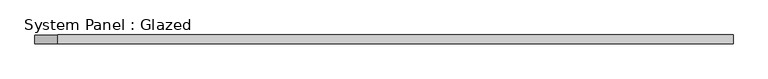
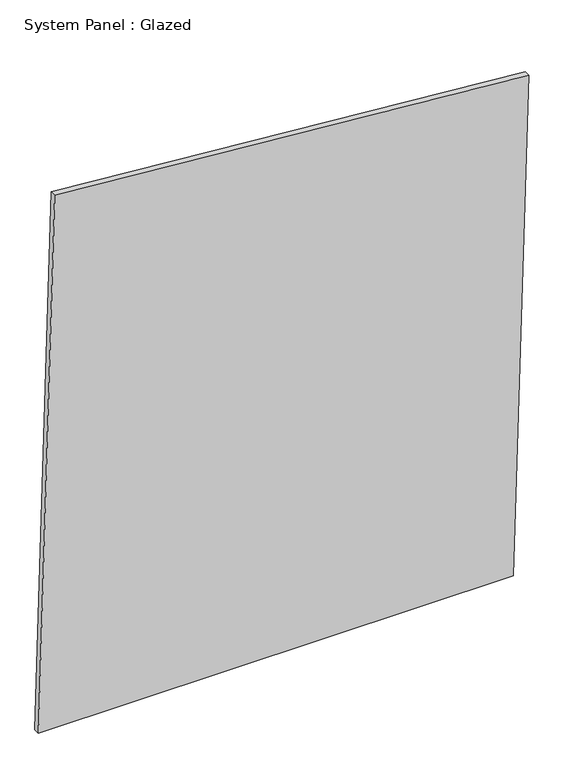
"""IFC4 building model written with IfcOpenShell, lengths in millimetres: plate geometry, System Panel : Glazed."""

import ifcopenshell
import ifcopenshell.guid

model = None  # the IFC model being written
_history = None  # IfcOwnerHistory: only IFC2X3 demands one
_inside = {}  # id of a spatial element -> (the spatial element, [elements in it])
_under = {}  # id of a project, library or spatial element -> (it, [spatial elements below it])
_declared = {}  # id of a project -> (the project, [libraries it declares])
_typed = {}  # id of a type object -> (the type object, [elements of that type])
_made_of = {}  # id of a material, layer set ... -> (it, [elements and type objects made of it])


def new_model(schema):
    """Start an empty IFC model of exactly this schema.

    Asked for "IFC4X3", IfcOpenShell would pick the latest addendum, in which some entities
    have other attributes; the version numbers below select the first issue.
    IFC2X3 requires an IfcOwnerHistory on every rooted entity: one is made here for all.
    """
    global model, _history
    if schema == "IFC4X3":
        model = ifcopenshell.file(schema_version=(4, 3, 0, 0))
    else:
        model = ifcopenshell.file(schema=schema)
    _inside.clear()
    _under.clear()
    _declared.clear()
    _typed.clear()
    _made_of.clear()
    _history = None
    if model.schema == "IFC2X3":
        org = make("IfcOrganization", Name="unknown")
        user = make(
            "IfcPersonAndOrganization",
            ThePerson=make("IfcPerson", FamilyName="unknown"),
            TheOrganization=org,
        )
        app = make(
            "IfcApplication",
            ApplicationDeveloper=org,
            Version="unknown",
            ApplicationFullName="unknown",
            ApplicationIdentifier="unknown",
        )
        _history = make(
            "IfcOwnerHistory",
            OwningUser=user,
            OwningApplication=app,
            ChangeAction="ADDED",
            CreationDate=0,
        )
    return model


def make(cls, **values):
    """One entity of the class cls with the attributes given. An attribute that is None is left unset."""
    return model.create_entity(
        cls, **{name: value for name, value in values.items() if value is not None}
    )


def rooted(cls, **values):
    """An entity with a GlobalId (a new one), such as an element, a storey or a relation."""
    return make(cls, GlobalId=ifcopenshell.guid.new(), OwnerHistory=_history, **values)


def si_unit(unit_type, name, prefix=None):
    """IfcSIUnit, for example si_unit("LENGTHUNIT", "METRE", prefix="MILLI")."""
    return make("IfcSIUnit", UnitType=unit_type, Prefix=prefix, Name=name)


def assignment(units):
    """IfcUnitAssignment: the units of a project."""
    return None if units is None else make("IfcUnitAssignment", Units=units)


def point(xyz):
    """IfcCartesianPoint."""
    return None if xyz is None else make("IfcCartesianPoint", Coordinates=xyz)


def direction(xyz):
    """IfcDirection."""
    return None if xyz is None else make("IfcDirection", DirectionRatios=xyz)


def frame(location, z_axis=None, x_axis=None):
    """IfcAxis2Placement3D, a coordinate frame: its origin and axes. An axis left out is left unset."""
    return make(
        "IfcAxis2Placement3D",
        Location=point(location),
        Axis=direction(z_axis),
        RefDirection=direction(x_axis),
    )


def origin():
    """The frame at (0, 0, 0) with its axes left unset."""
    return frame((0.0, 0.0, 0.0))


def place(relative_to, where):
    """IfcLocalPlacement: puts the frame where relative to a parent placement (None: the world)."""
    return make(
        "IfcLocalPlacement", PlacementRelTo=relative_to, RelativePlacement=where
    )


def context(
    kind, dimensions, precision=None, world=None, true_north=None, identifier=None
):
    """IfcGeometricRepresentationContext, for example the 3D "Model" context."""
    return make(
        "IfcGeometricRepresentationContext",
        ContextIdentifier=identifier,
        ContextType=kind,
        CoordinateSpaceDimension=dimensions,
        Precision=precision,
        WorldCoordinateSystem=world,
        TrueNorth=true_north,
    )


def project(units=None, contexts=None):
    """IfcProject with its units and contexts."""
    return rooted(
        "IfcProject",
        Name="project",
        RepresentationContexts=contexts,
        UnitsInContext=assignment(units),
    )


def spatial(cls, under=None, at=None, **own):
    """A site, building, storey or space (cls), placed at a placement, below another one or the project."""
    s = rooted(cls, ObjectPlacement=at, **own)
    if under is not None:
        _under.setdefault(under.id(), (under, []))[1].append(s)
    return s


def polyline(points):
    """IfcPolyline through the points."""
    return make("IfcPolyline", Points=[point(p) for p in points])


def outline(outer, holes=None, kind="AREA"):
    """IfcArbitraryClosedProfileDef: a profile drawn as a closed curve; with holes, ...WithVoids."""
    if holes is None:
        return make("IfcArbitraryClosedProfileDef", ProfileType=kind, OuterCurve=outer)
    return make(
        "IfcArbitraryProfileDefWithVoids",
        ProfileType=kind,
        OuterCurve=outer,
        InnerCurves=holes,
    )


def extrude(swept, where, along, depth):
    """IfcExtrudedAreaSolid: the profile swept, set in the frame where, extruded along a direction by depth."""
    return make(
        "IfcExtrudedAreaSolid",
        SweptArea=swept,
        Position=where,
        ExtrudedDirection=direction(along),
        Depth=depth,
    )


def shape(context_of_items, identifier, shape_type, items):
    """IfcShapeRepresentation: the items that make up one representation, for example the "Body"."""
    return make(
        "IfcShapeRepresentation",
        ContextOfItems=context_of_items,
        RepresentationIdentifier=identifier,
        RepresentationType=shape_type,
        Items=items,
    )


def source(mapping_origin, context_of_items, identifier, shape_type, items):
    """IfcRepresentationMap: a shape defined once, which mapped items show again and again."""
    return make(
        "IfcRepresentationMap",
        MappingOrigin=mapping_origin,
        MappedRepresentation=shape(context_of_items, identifier, shape_type, items),
    )


def transform(
    local_origin,
    x_axis=None,
    y_axis=None,
    z_axis=None,
    scale=None,
    scale2=None,
    scale3=None,
    uniform=True,
):
    """IfcCartesianTransformationOperator3D, or its non-uniform kind. x_axis, y_axis, z_axis: its Axis1, 2, 3."""
    if uniform:
        return make(
            "IfcCartesianTransformationOperator3D",
            Axis1=direction(x_axis),
            Axis2=direction(y_axis),
            LocalOrigin=point(local_origin),
            Scale=scale,
            Axis3=direction(z_axis),
        )
    return make(
        "IfcCartesianTransformationOperator3DnonUniform",
        Axis1=direction(x_axis),
        Axis2=direction(y_axis),
        LocalOrigin=point(local_origin),
        Scale=scale,
        Axis3=direction(z_axis),
        Scale2=scale2,
        Scale3=scale3,
    )


def mapped(mapping_source, mapping_target):
    """IfcMappedItem: shows the shape of a source again, moved by a transform."""
    return make(
        "IfcMappedItem", MappingSource=mapping_source, MappingTarget=mapping_target
    )


def made_of(thing, what):
    """Note that an element or type object is made of a material, layer set ...; save() writes the relation."""
    if what is not None:
        _made_of.setdefault(what.id(), (what, []))[1].append(thing)
    return thing


def element(
    cls,
    number,
    at=None,
    inside=None,
    cuts=None,
    type_object=None,
    material=None,
    context=None,
    identifier="Body",
    shape_type=None,
    held_by="IfcProductDefinitionShape",
    body=None,
    shapes=None,
    **own,
):
    """One element of the class cls, such as IfcWall. Its Tag is "e" and its number.

    at: its placement. inside: the storey or other place that contains it. cuts: it is an
    opening in that element (IfcRelVoidsElement). A single representation is given by context,
    identifier, shape_type and body (its items); several are given by shapes. held_by: the class
    of the entity that holds the representations. save() writes the other relations.
    """
    e = rooted(cls, Tag="e%d" % number, ObjectPlacement=at, **own)
    if body is not None:
        shapes = [shape(context, identifier, shape_type, body)]
    if shapes is not None:
        e.Representation = make(held_by, Representations=shapes)
    if inside is not None:
        _inside.setdefault(inside.id(), (inside, []))[1].append(e)
    if cuts is not None:
        rooted(
            "IfcRelVoidsElement", RelatingBuildingElement=cuts, RelatedOpeningElement=e
        )
    if type_object is not None:
        _typed.setdefault(type_object.id(), (type_object, []))[1].append(e)
    return made_of(e, material)


def aggregate(whole, parts):
    """IfcRelAggregates: a whole, such as a stair, and the parts it consists of."""
    return rooted("IfcRelAggregates", RelatingObject=whole, RelatedObjects=parts)


def save(model, path):
    """Write the relations noted so far, then the file.

    IfcRelAggregates (storeys below a building ...), IfcRelContainedInSpatialStructure (elements
    in a storey), IfcRelDefinesByType, IfcRelAssociatesMaterial and IfcRelDeclares: one each for
    every whole, place, type object, material and project.
    """
    for whole, parts in _under.values():
        aggregate(whole, parts)
    for where, things in _inside.values():
        rooted(
            "IfcRelContainedInSpatialStructure",
            RelatedElements=things,
            RelatingStructure=where,
        )
    for kind, things in _typed.values():
        rooted("IfcRelDefinesByType", RelatedObjects=things, RelatingType=kind)
    for what, things in _made_of.values():
        rooted("IfcRelAssociatesMaterial", RelatedObjects=things, RelatingMaterial=what)
    for by, libraries in _declared.values():
        rooted("IfcRelDeclares", RelatingContext=by, RelatedDefinitions=libraries)
    model.write(path)


def system_panel_glazed_15b89219(model_context):
    return source(origin(), model_context, "Body", "SweptSolid", [
        extrude(outline(polyline([(0.0, -1007.0351176), (0.0, 942.9445704), (2151.1749822, 1007.0351176), (2310.4173325, -940.4629834), (0.0, -1007.0351176)])), frame((0.0, -49.5, 0.0), z_axis=(0.0, 1.0, 0.0), x_axis=(0.0, 0.0, 1.0)), (0.0, 0.0, 1.0), 25.0),
    ])


if __name__ == "__main__":
    model = new_model("IFC4")
    model_context = context("Model", 3, world=origin())
    ifc_project = project(units=[si_unit("LENGTHUNIT", "METRE", prefix="MILLI")], contexts=[model_context])
    site = spatial("IfcSite", under=ifc_project)
    building = spatial("IfcBuilding", under=site)
    placement = place(None, origin())
    system_panel_glazed_shape = system_panel_glazed_15b89219(model_context)
    element("IfcPlate", 1, ObjectType="System Panel : Glazed", at=placement, inside=building, context=model_context, shape_type="MappedRepresentation", body=[
        mapped(system_panel_glazed_shape, transform((0.0, 0.0, 0.0), x_axis=(1.0, 0.0, 0.0), y_axis=(0.0, 1.0, 0.0), z_axis=(0.0, 0.0, 1.0))),
    ])
    save(model, "model.ifc")

# Revit data of these elements
# Element 1 (IfcPlate, "System Panel : Glazed")
#   Materials on its faces: "Glass, Clear Glazing"
# Materials
#   "Glass, Clear Glazing": class "Glass", colour RGB 247 249 248, transparency 0.85, Description = "Clear glazing", Cost = 0
